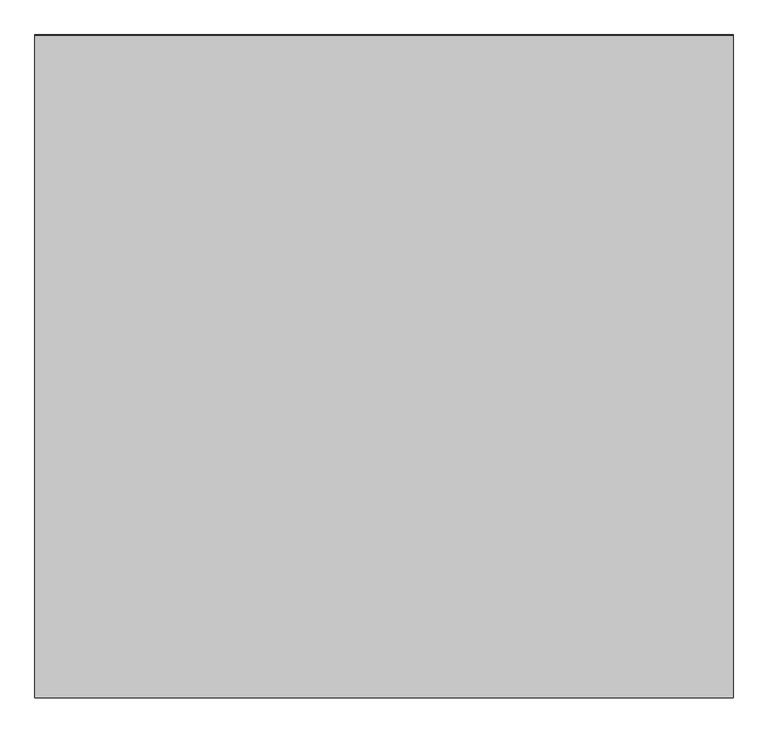
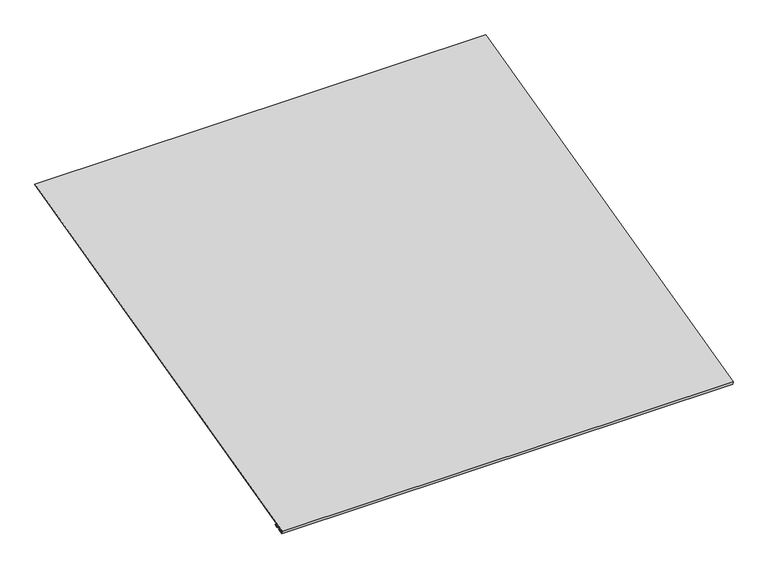
"""IFC4 building model written with IfcOpenShell, lengths in millimetres: proxy geometry, Gutter @ Roof : Gutter @ Roof."""

from ifc_helpers import new_model, si_unit, frame, origin, place, context, project, spatial, polyline, outline, extrude, source, transform, mapped, element, save


def generic_models_64ebdc1b(model_context):
    return source(origin(), model_context, "Body", "SweptSolid", [
        extrude(outline(polyline([(-5251.6312056, 42833.0279403), (-5255.0603039, 42846.7443334), (-3355.5418975, 43321.623935), (-3354.925857, 43319.159773), (-5251.9801014, 42844.8962119), (-5249.7880003, 42836.1278074), (-5230.2696218, 42841.1725723), (-5229.6340146, 42838.7133847), (-5251.6312056, 42833.0279403)])), frame((12382.7678845, 0.0, 0.0), z_axis=(1.0, 0.0, 0.0), x_axis=(0.0, 1.0, 0.0)), (0.0, 0.0, 1.0), 2000.25),
        extrude(outline(polyline([(-5213.885254, 42839.191407), (-5228.0455647, 42844.1599484), (-5244.095215, 42840.011719), (-5244.7308223, 42842.4709066), (-5227.9333922, 42846.8124088), (-5213.7670506, 42841.8417513), (-5200.4128381, 42845.2277164), (-5199.788574, 42842.765625), (-5213.885254, 42839.191407)])), frame((12382.7678845, 0.0, 0.0), z_axis=(1.0, 0.0, 0.0), x_axis=(0.0, 1.0, 0.0)), (0.0, 0.0, 1.0), 2000.25),
    ])


if __name__ == "__main__":
    model = new_model("IFC4")
    model_context = context("Model", 3, world=origin())
    ifc_project = project(units=[si_unit("LENGTHUNIT", "METRE", prefix="MILLI")], contexts=[model_context])
    site = spatial("IfcSite", under=ifc_project)
    building = spatial("IfcBuilding", under=site)
    placement = place(None, origin())
    generic_models_shape = generic_models_64ebdc1b(model_context)
    element("IfcBuildingElementProxy", 1, Name="Gutter @ Roof : Gutter @ Roof", ObjectType="Gutter @ Roof : Gutter @ Roof", at=placement, inside=building, context=model_context, shape_type="MappedRepresentation", body=[
        mapped(generic_models_shape, transform((0.0, 0.0, 0.0), x_axis=(1.0, 0.0, 0.0), y_axis=(0.0, 1.0, 0.0), z_axis=(0.0, 0.0, 1.0))),
    ])
    save(model, "model.ifc")

# Revit data of these elements
# Type "Gutter @ Roof : Gutter @ Roof"
#   NameOverride = "Gutter @ Roof"
# Element 1 (IfcBuildingElementProxy, "Gutter @ Roof : Gutter @ Roof")
#   Materials on its faces: "CONT. SEAMLESS 16 GA COPPER BRAKE METAL GUTTER"
# Materials
#   "CONT. SEAMLESS 16 GA COPPER BRAKE METAL GUTTER": class "Unassigned", colour RGB 128 128 128, transparency 0
